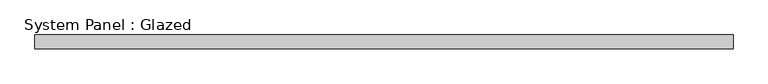
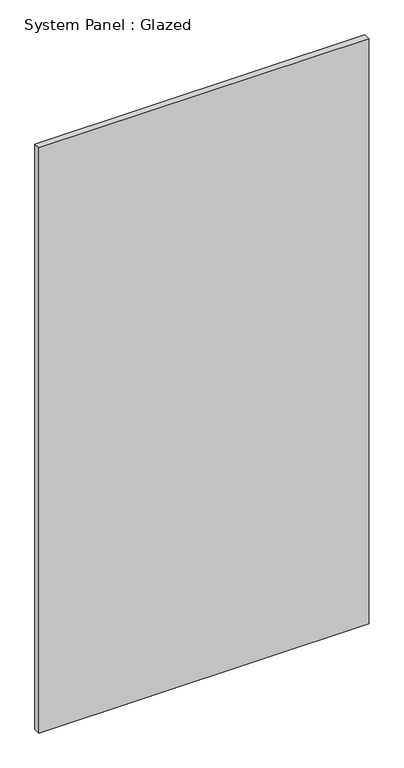
"""IFC4 building model written with IfcOpenShell, lengths in millimetres: plate geometry, System Panel : Glazed."""

import ifcopenshell
import ifcopenshell.guid

model = None  # the IFC model being written
_history = None  # IfcOwnerHistory: only IFC2X3 demands one
_inside = {}  # id of a spatial element -> (the spatial element, [elements in it])
_under = {}  # id of a project, library or spatial element -> (it, [spatial elements below it])
_declared = {}  # id of a project -> (the project, [libraries it declares])
_typed = {}  # id of a type object -> (the type object, [elements of that type])
_made_of = {}  # id of a material, layer set ... -> (it, [elements and type objects made of it])


def new_model(schema):
    """Start an empty IFC model of exactly this schema.

    Asked for "IFC4X3", IfcOpenShell would pick the latest addendum, in which some entities
    have other attributes; the version numbers below select the first issue.
    IFC2X3 requires an IfcOwnerHistory on every rooted entity: one is made here for all.
    """
    global model, _history
    if schema == "IFC4X3":
        model = ifcopenshell.file(schema_version=(4, 3, 0, 0))
    else:
        model = ifcopenshell.file(schema=schema)
    _inside.clear()
    _under.clear()
    _declared.clear()
    _typed.clear()
    _made_of.clear()
    _history = None
    if model.schema == "IFC2X3":
        org = make("IfcOrganization", Name="unknown")
        user = make(
            "IfcPersonAndOrganization",
            ThePerson=make("IfcPerson", FamilyName="unknown"),
            TheOrganization=org,
        )
        app = make(
            "IfcApplication",
            ApplicationDeveloper=org,
            Version="unknown",
            ApplicationFullName="unknown",
            ApplicationIdentifier="unknown",
        )
        _history = make(
            "IfcOwnerHistory",
            OwningUser=user,
            OwningApplication=app,
            ChangeAction="ADDED",
            CreationDate=0,
        )
    return model


def make(cls, **values):
    """One entity of the class cls with the attributes given. An attribute that is None is left unset."""
    return model.create_entity(
        cls, **{name: value for name, value in values.items() if value is not None}
    )


def rooted(cls, **values):
    """An entity with a GlobalId (a new one), such as an element, a storey or a relation."""
    return make(cls, GlobalId=ifcopenshell.guid.new(), OwnerHistory=_history, **values)


def si_unit(unit_type, name, prefix=None):
    """IfcSIUnit, for example si_unit("LENGTHUNIT", "METRE", prefix="MILLI")."""
    return make("IfcSIUnit", UnitType=unit_type, Prefix=prefix, Name=name)


def assignment(units):
    """IfcUnitAssignment: the units of a project."""
    return None if units is None else make("IfcUnitAssignment", Units=units)


def point(xyz):
    """IfcCartesianPoint."""
    return None if xyz is None else make("IfcCartesianPoint", Coordinates=xyz)


def direction(xyz):
    """IfcDirection."""
    return None if xyz is None else make("IfcDirection", DirectionRatios=xyz)


def frame(location, z_axis=None, x_axis=None):
    """IfcAxis2Placement3D, a coordinate frame: its origin and axes. An axis left out is left unset."""
    return make(
        "IfcAxis2Placement3D",
        Location=point(location),
        Axis=direction(z_axis),
        RefDirection=direction(x_axis),
    )


def origin():
    """The frame at (0, 0, 0) with its axes left unset."""
    return frame((0.0, 0.0, 0.0))


def origin_with_axes():
    """The frame at (0, 0, 0) with the z axis (0, 0, 1) and the x axis (1, 0, 0) written out."""
    return frame((0.0, 0.0, 0.0), z_axis=(0.0, 0.0, 1.0), x_axis=(1.0, 0.0, 0.0))


def place(relative_to, where):
    """IfcLocalPlacement: puts the frame where relative to a parent placement (None: the world)."""
    return make(
        "IfcLocalPlacement", PlacementRelTo=relative_to, RelativePlacement=where
    )


def context(
    kind, dimensions, precision=None, world=None, true_north=None, identifier=None
):
    """IfcGeometricRepresentationContext, for example the 3D "Model" context."""
    return make(
        "IfcGeometricRepresentationContext",
        ContextIdentifier=identifier,
        ContextType=kind,
        CoordinateSpaceDimension=dimensions,
        Precision=precision,
        WorldCoordinateSystem=world,
        TrueNorth=true_north,
    )


def project(units=None, contexts=None):
    """IfcProject with its units and contexts."""
    return rooted(
        "IfcProject",
        Name="project",
        RepresentationContexts=contexts,
        UnitsInContext=assignment(units),
    )


def spatial(cls, under=None, at=None, **own):
    """A site, building, storey or space (cls), placed at a placement, below another one or the project."""
    s = rooted(cls, ObjectPlacement=at, **own)
    if under is not None:
        _under.setdefault(under.id(), (under, []))[1].append(s)
    return s


def polyline(points):
    """IfcPolyline through the points."""
    return make("IfcPolyline", Points=[point(p) for p in points])


def outline(outer, holes=None, kind="AREA"):
    """IfcArbitraryClosedProfileDef: a profile drawn as a closed curve; with holes, ...WithVoids."""
    if holes is None:
        return make("IfcArbitraryClosedProfileDef", ProfileType=kind, OuterCurve=outer)
    return make(
        "IfcArbitraryProfileDefWithVoids",
        ProfileType=kind,
        OuterCurve=outer,
        InnerCurves=holes,
    )


def extrude(swept, where, along, depth):
    """IfcExtrudedAreaSolid: the profile swept, set in the frame where, extruded along a direction by depth."""
    return make(
        "IfcExtrudedAreaSolid",
        SweptArea=swept,
        Position=where,
        ExtrudedDirection=direction(along),
        Depth=depth,
    )


def shape(context_of_items, identifier, shape_type, items):
    """IfcShapeRepresentation: the items that make up one representation, for example the "Body"."""
    return make(
        "IfcShapeRepresentation",
        ContextOfItems=context_of_items,
        RepresentationIdentifier=identifier,
        RepresentationType=shape_type,
        Items=items,
    )


def source(mapping_origin, context_of_items, identifier, shape_type, items):
    """IfcRepresentationMap: a shape defined once, which mapped items show again and again."""
    return make(
        "IfcRepresentationMap",
        MappingOrigin=mapping_origin,
        MappedRepresentation=shape(context_of_items, identifier, shape_type, items),
    )


def transform(
    local_origin,
    x_axis=None,
    y_axis=None,
    z_axis=None,
    scale=None,
    scale2=None,
    scale3=None,
    uniform=True,
):
    """IfcCartesianTransformationOperator3D, or its non-uniform kind. x_axis, y_axis, z_axis: its Axis1, 2, 3."""
    if uniform:
        return make(
            "IfcCartesianTransformationOperator3D",
            Axis1=direction(x_axis),
            Axis2=direction(y_axis),
            LocalOrigin=point(local_origin),
            Scale=scale,
            Axis3=direction(z_axis),
        )
    return make(
        "IfcCartesianTransformationOperator3DnonUniform",
        Axis1=direction(x_axis),
        Axis2=direction(y_axis),
        LocalOrigin=point(local_origin),
        Scale=scale,
        Axis3=direction(z_axis),
        Scale2=scale2,
        Scale3=scale3,
    )


def mapped(mapping_source, mapping_target):
    """IfcMappedItem: shows the shape of a source again, moved by a transform."""
    return make(
        "IfcMappedItem", MappingSource=mapping_source, MappingTarget=mapping_target
    )


def made_of(thing, what):
    """Note that an element or type object is made of a material, layer set ...; save() writes the relation."""
    if what is not None:
        _made_of.setdefault(what.id(), (what, []))[1].append(thing)
    return thing


def element(
    cls,
    number,
    at=None,
    inside=None,
    cuts=None,
    type_object=None,
    material=None,
    context=None,
    identifier="Body",
    shape_type=None,
    held_by="IfcProductDefinitionShape",
    body=None,
    shapes=None,
    **own,
):
    """One element of the class cls, such as IfcWall. Its Tag is "e" and its number.

    at: its placement. inside: the storey or other place that contains it. cuts: it is an
    opening in that element (IfcRelVoidsElement). A single representation is given by context,
    identifier, shape_type and body (its items); several are given by shapes. held_by: the class
    of the entity that holds the representations. save() writes the other relations.
    """
    e = rooted(cls, Tag="e%d" % number, ObjectPlacement=at, **own)
    if body is not None:
        shapes = [shape(context, identifier, shape_type, body)]
    if shapes is not None:
        e.Representation = make(held_by, Representations=shapes)
    if inside is not None:
        _inside.setdefault(inside.id(), (inside, []))[1].append(e)
    if cuts is not None:
        rooted(
            "IfcRelVoidsElement", RelatingBuildingElement=cuts, RelatedOpeningElement=e
        )
    if type_object is not None:
        _typed.setdefault(type_object.id(), (type_object, []))[1].append(e)
    return made_of(e, material)


def aggregate(whole, parts):
    """IfcRelAggregates: a whole, such as a stair, and the parts it consists of."""
    return rooted("IfcRelAggregates", RelatingObject=whole, RelatedObjects=parts)


def save(model, path):
    """Write the relations noted so far, then the file.

    IfcRelAggregates (storeys below a building ...), IfcRelContainedInSpatialStructure (elements
    in a storey), IfcRelDefinesByType, IfcRelAssociatesMaterial and IfcRelDeclares: one each for
    every whole, place, type object, material and project.
    """
    for whole, parts in _under.values():
        aggregate(whole, parts)
    for where, things in _inside.values():
        rooted(
            "IfcRelContainedInSpatialStructure",
            RelatedElements=things,
            RelatingStructure=where,
        )
    for kind, things in _typed.values():
        rooted("IfcRelDefinesByType", RelatedObjects=things, RelatingType=kind)
    for what, things in _made_of.values():
        rooted("IfcRelAssociatesMaterial", RelatedObjects=things, RelatingMaterial=what)
    for by, libraries in _declared.values():
        rooted("IfcRelDeclares", RelatingContext=by, RelatedDefinitions=libraries)
    model.write(path)


def system_panel_glazed_eec4e8b3(model_context):
    return source(origin(), model_context, "Body", "SweptSolid", [
        extrude(outline(polyline([(626.7857144, 24.5), (-626.7857144, 24.5), (-626.7857144, 49.5), (626.7857144, 49.5), (626.7857144, 24.5)])), origin_with_axes(), (0.0, 0.0, 1.0), 2350.0),
    ])


if __name__ == "__main__":
    model = new_model("IFC4")
    model_context = context("Model", 3, world=origin())
    ifc_project = project(units=[si_unit("LENGTHUNIT", "METRE", prefix="MILLI")], contexts=[model_context])
    site = spatial("IfcSite", under=ifc_project)
    building = spatial("IfcBuilding", under=site)
    placement = place(None, origin())
    system_panel_glazed_shape = system_panel_glazed_eec4e8b3(model_context)
    element("IfcPlate", 1, ObjectType="System Panel : Glazed", at=placement, inside=building, context=model_context, shape_type="MappedRepresentation", body=[
        mapped(system_panel_glazed_shape, transform((0.0, 0.0, 0.0), x_axis=(1.0, 0.0, 0.0), y_axis=(0.0, 1.0, 0.0), z_axis=(0.0, 0.0, 1.0))),
    ])
    save(model, "model.ifc")

# Revit data of these elements
# Type "System Panel : Glazed"
#   Construction Type Id = "GSP4R"
#   Analytic Construction = "1/8 in Pilkington single glazing"
#   Visual Light Transmittance = 0.9
#   Solar Heat Gain Coefficient = 0.86
#   Heat Transfer Coefficient (U) = 6.7069 W/(m²·K)
#   Define Thermal Properties by = 1
# Element 1 (IfcPlate, "System Panel : Glazed")
#   Materials on its faces: "Glass"
# Materials
#   "Glass": class "Glass", colour RGB 0 128 192, transparency 0.75, Description = "Soda Lime Glass", Cost = 0
